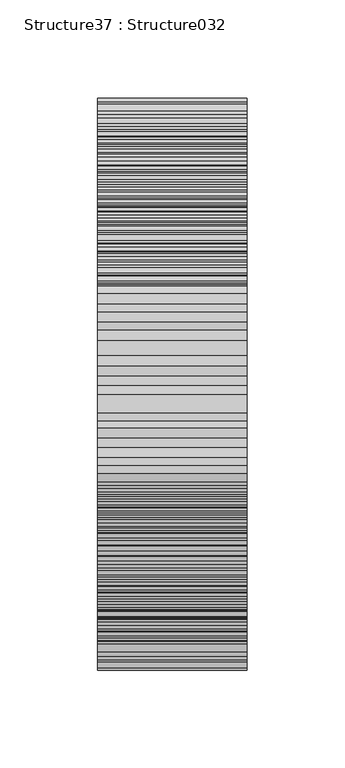
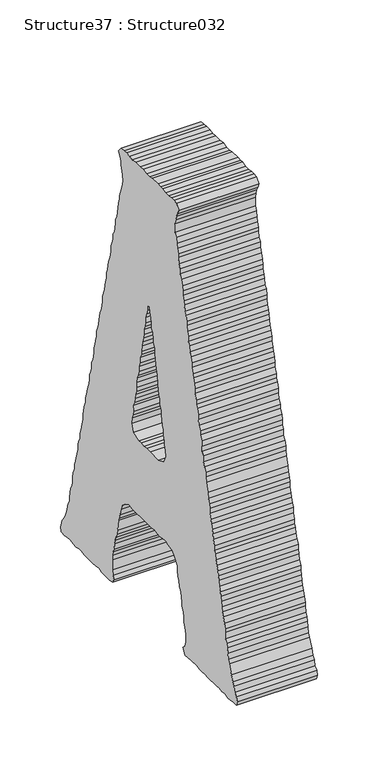
"""IFC4 building model written with IfcOpenShell, lengths in millimetres: proxy geometry, Structure37 : Structure032."""

from ifc_helpers import new_model, si_unit, frame, origin, place, context, project, spatial, polyline, outline, extrude, source, transform, mapped, element, save


def structure37_structure032_6acbcdab(model_context):
    return source(origin(), model_context, "Body", "SweptSolid", [
        extrude(outline(polyline([(258437.7580543, 3818.8310229), (258440.1200321, 3824.1149855), (258440.6992943, 3828.2163546), (258441.301021, 3833.4730389), (258443.0388077, 3838.1761347), (258443.6180699, 3841.6741725), (258445.3799256, 3846.9757858), (258445.3799256, 3851.6612309), (258447.1401768, 3856.9179152), (258448.3211657, 3861.0192843), (258449.5021546, 3866.3032469), (258450.660679, 3870.4030114), (258451.2399413, 3875.0772243), (258453.001797, 3878.5784713), (258453.5810592, 3884.4609514), (258453.5810592, 3888.5623205), (258454.7620481, 3893.822214), (258456.5222993, 3896.763454), (258457.6808237, 3902.6314927), (258458.8618126, 3906.1487857), (258460.0219417, 3910.8310217), (258460.0219417, 3915.5068392), (258461.2029306, 3919.6066036), (258462.9631817, 3924.8905662), (258464.7009684, 3929.5904528), (258464.7009684, 3934.8503464), (258466.4612195, 3938.3499888), (258467.643813, 3944.235678), (258467.643813, 3947.7337158), (258469.4040641, 3952.435207), (258470.0057908, 3957.1190475), (258471.1643153, 3962.3757319), (258472.9245664, 3966.5043792), (258472.9245664, 3974.7055128), (258471.766042, 3979.3781211), (258470.5850531, 3984.0635662), (258468.8248019, 3987.5792547), (258466.4612195, 3992.2614906), (258470.5850531, 3996.9645864), (258474.6848175, 3997.5486624), (258478.7861866, 3997.5486624), (258484.0685446, 3996.390138), (258488.7475713, 3996.390138), (258494.0299293, 3997.5486624), (258497.5295717, 3996.9645864), (258501.6518007, 3997.5486624), (258511.0114587, 3997.5486624), (258515.69209, 3996.390138), (258520.3727213, 3996.390138), (258525.6534747, 3997.5486624), (258530.9358327, 3996.9645864), (258538.5577041, 3996.9645864), (258543.8175976, 3996.390138), (258547.9173621, 3997.5486624), (258553.1997201, 3997.5486624), (258557.3010892, 3996.9645864), (258562.5593781, 3996.390138), (258566.081485, 3991.6806238), (258563.740367, 3987.5792547), (258562.5593781, 3983.4794902), (258562.0025804, 3979.9621971), (258560.8215915, 3974.7055128), (258559.0613403, 3965.8930249), (258560.2423292, 3961.794865), (258561.4008537, 3956.5349715), (258564.9004961, 3947.1496398), (258564.9004961, 3944.235678), (258566.081485, 3938.9517154), (258567.2624739, 3934.2758979), (258567.8417361, 3928.9919353), (258569.022725, 3924.2888396), (258571.3622384, 3919.6066036), (258571.3622384, 3916.0909152), (258571.9431052, 3910.8310217), (258573.1240941, 3906.1487857), (258575.4636075, 3902.6314927), (258575.4636075, 3897.3475301), (258577.2013942, 3892.6636896), (258578.3823831, 3888.5623205), (258578.3823831, 3883.8881076), (258579.5649766, 3878.5784713), (258581.3252277, 3873.9203044), (258583.0854788, 3869.8189354), (258583.6647411, 3866.3032469), (258584.2664678, 3861.0192843), (258586.0042544, 3856.9179152), (258586.0042544, 3851.6612309), (258587.7661102, 3846.9757858), (258588.3453724, 3842.8583706), (258589.5263613, 3837.6000817), (258592.4451369, 3829.374879), (258592.4451369, 3824.1149855), (258593.6261258, 3820.015221), (258594.7862548, 3815.3313805), (258597.1482326, 3810.0474179), (258597.7274949, 3806.5317294), (258598.9084838, 3801.8462843), (258599.487746, 3797.1463977), (258601.2271373, 3791.8865042), (258602.4081262, 3788.3611881), (258602.4081262, 3783.0868532), (258604.1683773, 3777.8285642), (258604.770104, 3774.3032481), (258606.5303551, 3769.0176809), (258607.0871529, 3764.3611187), (258607.6664151, 3759.6596275), (258608.8490086, 3756.1423345), (258610.6092598, 3751.4424479), (258611.2109864, 3745.6000829), (258612.3695109, 3740.9162424), (258614.129762, 3737.9750024), (258614.129762, 3732.7167134), (258615.2882865, 3727.4311462), (258617.0501422, 3723.3313817), (258618.2311311, 3718.0554422), (258619.41212, 3714.5301261), (258620.5931089, 3710.4560353), (258620.5931089, 3705.7545441), (258622.9101578, 3699.8881101), (258624.0927513, 3695.2122926), (258624.6720136, 3691.0868544), (258624.6720136, 3686.4030139), (258625.8530025, 3682.8857208), (258627.6132536, 3677.0449605), (258628.1925158, 3673.5276674), (258629.9303025, 3668.8261762), (258629.9303025, 3663.5598643), (258632.2938849, 3659.4584952), (258633.4748738, 3655.3587307), (258633.4748738, 3650.6845178), (258634.6333983, 3645.4262289), (258636.3936494, 3640.114988), (258637.5521739, 3636.0408972), (258638.7347674, 3632.5155811), (258639.3140296, 3627.2396415), (258641.0742807, 3622.555801), (258642.2552696, 3617.2718384), (258642.2552696, 3612.5976255), (258642.8569963, 3608.4705827), (258645.1740452, 3604.3964919), (258646.3566387, 3599.1125293), (258647.5376276, 3594.4286888), (258647.5376276, 3590.3289243), (258649.2978788, 3586.2115092), (258652.1941899, 3576.2693797), (258653.9785101, 3572.1423369), (258655.7387612, 3568.6426945), (258659.2592635, 3563.366755), (258660.4177879, 3560.441561), (258662.1796436, 3555.1848766), (258660.9986547, 3551.0658569), (258655.1370345, 3550.4833855), (258651.6373921, 3551.0658569), (258646.3566387, 3551.6675836), (258641.6760074, 3550.4833855), (258636.3936494, 3550.4833855), (258631.7146227, 3551.6675836), (258627.6132536, 3551.6675836), (258622.9101578, 3551.0658569), (258618.8103933, 3551.0658569), (258612.9712376, 3550.4833855), (258608.8490086, 3550.4833855), (258604.1683773, 3551.0658569), (258598.9084838, 3551.6675836), (258594.7862548, 3550.4833855), (258581.3252277, 3550.4833855), (258576.0428697, 3551.6675836), (258573.7033564, 3555.7416744), (258575.4636075, 3559.2669905), (258576.6445964, 3563.9412034), (258576.6445964, 3573.9266571), (258576.6445964, 3578.6104977), (258575.4636075, 3582.7102621), (258573.7033564, 3586.2115092), (258573.1240941, 3592.0955938), (258571.9431052, 3596.1953583), (258570.1812495, 3600.2967274), (258569.022725, 3604.3964919), (258567.8417361, 3609.0723094), (258566.6832117, 3619.6145609), (258565.5022228, 3622.555801), (258563.740367, 3627.2396415), (258562.5593781, 3633.0980525), (258559.6406026, 3638.9580681), (258555.5392335, 3642.4833842), (258549.098351, 3645.9830266), (258544.4193243, 3644.8245022), (258535.0372018, 3644.8245022), (258529.1755816, 3645.4262289), (258516.8730789, 3645.4262289), (258511.5907209, 3644.8245022), (258507.4909565, 3645.9830266), (258502.7878607, 3645.4262289), (258498.108834, 3644.8245022), (258494.0299293, 3645.4262289), (258488.1458447, 3645.9830266), (258484.6478069, 3644.8245022), (258477.6051977, 3643.0578326), (258474.0830909, 3639.5405396), (258469.4040641, 3633.0980525), (258469.4040641, 3627.8397636), (258468.2455397, 3622.555801), (258466.4612195, 3619.6145609), (258465.8819573, 3613.772196), (258463.5649084, 3610.2292293), (258462.3839195, 3604.9709403), (258461.8046573, 3601.4536473), (258461.8046573, 3596.7698067), (258459.4410748, 3592.0955938), (258458.8618126, 3587.3860796), (258458.2600859, 3582.7102621), (258456.5222993, 3578.6104977), (258454.7620481, 3572.7440636), (258455.3413103, 3565.1254015), (258457.1015615, 3559.2669905), (258460.0219417, 3556.3417965), (258456.5222993, 3550.4833855), (258451.2399413, 3551.0658569), (258446.5609145, 3551.6675836), (258437.1771875, 3551.6675836), (258432.4981607, 3551.0658569), (258427.795065, 3551.0658569), (258423.7177649, 3551.6675836), (258419.6163959, 3551.0658569), (258413.7323112, 3551.0658569), (258410.2342734, 3551.6675836), (258404.3726531, 3551.0658569), (258400.8521509, 3551.6675836), (258396.1715196, 3550.4833855), (258390.8891616, 3551.6675836), (258385.629268, 3550.4833855), (258381.5295035, 3551.0658569), (258376.8264078, 3551.6675836), (258372.1473811, 3551.6675836), (258370.3855253, 3556.3417965), (258371.5681188, 3560.441561), (258374.5093589, 3563.366755), (258375.6454189, 3568.6426945), (258377.40567, 3572.1423369), (258379.7692524, 3577.4535778), (258383.8465524, 3586.2115092), (258385.0275413, 3589.7544759), (258385.629268, 3595.5872132), (258386.7893971, 3600.2967274), (258387.970386, 3604.3964919), (258389.7081727, 3607.8961343), (258390.3098993, 3613.772196), (258390.3098993, 3617.2718384), (258391.4684238, 3622.555801), (258393.2302795, 3627.8397636), (258394.9905307, 3631.915459), (258396.1715196, 3636.0408972), (258396.7732463, 3641.2991861), (258397.330044, 3645.9830266), (258397.9093062, 3650.1004418), (258400.2712841, 3654.1841602), (258400.8521509, 3660.0682449), (258401.4538776, 3664.1423357), (258402.0331398, 3668.8261762), (258403.7933909, 3672.9435914), (258405.5311776, 3677.6274319), (258406.7121665, 3682.8857208), (258407.8931554, 3685.8285655), (258407.8931554, 3690.512406), (258409.6550111, 3695.786741), (258410.2342734, 3701.0723082), (258411.4152623, 3704.5879966), (258413.1530489, 3709.2718371), (258413.7323112, 3713.3555556), (258415.4941669, 3718.6571688), (258415.4941669, 3723.3313817), (258416.6751558, 3727.4311462), (258417.8561447, 3732.1149867), (258419.0371336, 3737.400554), (258421.3541825, 3746.1745313), (258422.5351714, 3750.8583719), (258422.5351714, 3755.559863), (258424.2970272, 3759.6596275), (258426.0572783, 3763.759392), (258426.0572783, 3769.6274306), (258428.3743272, 3773.11905), (258428.3743272, 3777.8285642), (258428.9760539, 3783.0868532), (258431.3171718, 3787.7867397), (258431.3171718, 3791.8865042), (258433.6791497, 3795.960595), (258434.2584119, 3801.8462843), (258434.2584119, 3805.9476534), (258436.5979252, 3811.2043377), (258437.7580543, 3814.7296538), (258437.7580543, 3818.8310229)]), holes=[polyline([(258500.4708118, 3720.4158154), (258513.9318389, 3720.4158154), (258519.2125923, 3720.9726131), (258524.4949503, 3719.8140887), (258528.5963194, 3720.9726131), (258532.6736194, 3720.4158154), (258541.4764797, 3723.3313817), (258544.4193243, 3730.9323932), (258543.2383354, 3736.7988273), (258542.0573465, 3740.9162424), (258540.874753, 3744.9999608), (258541.4764797, 3750.8583719), (258539.1369663, 3754.9854146), (258538.5577041, 3759.6596275), (258537.9559774, 3763.759392), (258536.1957263, 3767.8607611), (258535.6164641, 3772.5606477), (258535.6164641, 3777.2444882), (258535.0372018, 3782.5027771), (258533.2753461, 3786.0280932), (258532.0943572, 3790.7039107), (258532.0943572, 3795.4037973), (258529.7548438, 3800.6717138), (258529.7548438, 3805.9476534), (258527.9945927, 3810.0474179), (258527.4153305, 3813.5743386), (258526.8136038, 3819.4150989), (258525.6534747, 3824.1149855), (258524.4949503, 3828.790803), (258523.9156881, 3832.8921721), (258523.9156881, 3837.6000817), (258521.5537103, 3842.2758992), (258520.974448, 3846.3772683), (258520.974448, 3851.6612309), (258519.2125923, 3856.3161885), (258518.0316034, 3860.4432313), (258518.0316034, 3864.5446004), (258516.2938167, 3865.1190488), (258515.1128278, 3860.4432313), (258513.3525767, 3855.7353217), (258512.7733145, 3851.0595042), (258512.7733145, 3845.8012153), (258510.409732, 3842.2758992), (258509.8304698, 3836.9919366), (258509.8304698, 3833.4730389), (258507.4909565, 3828.790803), (258506.9116942, 3822.932392), (258506.332432, 3818.8310229), (258505.1514431, 3814.7296538), (258504.5497164, 3810.0474179), (258502.7878607, 3804.7730829), (258502.2085985, 3795.4037973), (258501.050074, 3790.7039107), (258500.4708118, 3786.0280932), (258498.7105607, 3783.0868532), (258498.7105607, 3777.8285642), (258496.3469782, 3773.11905), (258496.3469782, 3768.4432325), (258495.1884538, 3764.3611187), (258494.6091916, 3759.0595054), (258492.8489404, 3755.559863), (258492.8489404, 3750.3015741), (258491.0886893, 3744.9999608), (258491.0886893, 3741.5003184), (258489.9077004, 3736.7988273), (258488.7475713, 3730.9323932), (258492.2696782, 3723.9154578), (258500.4708118, 3720.4158154)])]), frame((-38594.2176606, 0.0, 0.0), z_axis=(1.0, 0.0, 0.0), x_axis=(0.0, 1.0, 0.0)), (0.0, 0.0, 1.0), 76.2),
    ])


if __name__ == "__main__":
    model = new_model("IFC4")
    model_context = context("Model", 3, world=origin())
    ifc_project = project(units=[si_unit("LENGTHUNIT", "METRE", prefix="MILLI")], contexts=[model_context])
    site = spatial("IfcSite", under=ifc_project)
    building = spatial("IfcBuilding", under=site)
    placement = place(None, origin())
    structure37_structure032_shape = structure37_structure032_6acbcdab(model_context)
    element("IfcBuildingElementProxy", 1, Name="Structure37 : Structure032", ObjectType="Structure37 : Structure032", at=placement, inside=building, context=model_context, shape_type="MappedRepresentation", body=[
        mapped(structure37_structure032_shape, transform((0.0, 0.0, 0.0), x_axis=(1.0, 0.0, 0.0), y_axis=(0.0, 1.0, 0.0), z_axis=(0.0, 0.0, 1.0))),
    ])
    save(model, "model.ifc")

# Revit data of these elements
# Type "Structure37 : Structure032"
#   NameOverride = "Structure032"
# Element 1 (IfcBuildingElementProxy, "Structure37 : Structure032")
#   Materials on its faces: "BRUSHED ALUM. LETTERING"
# Materials
#   "BRUSHED ALUM. LETTERING": class "Unassigned", colour RGB 169 181 186, transparency 0, Cost = 0
